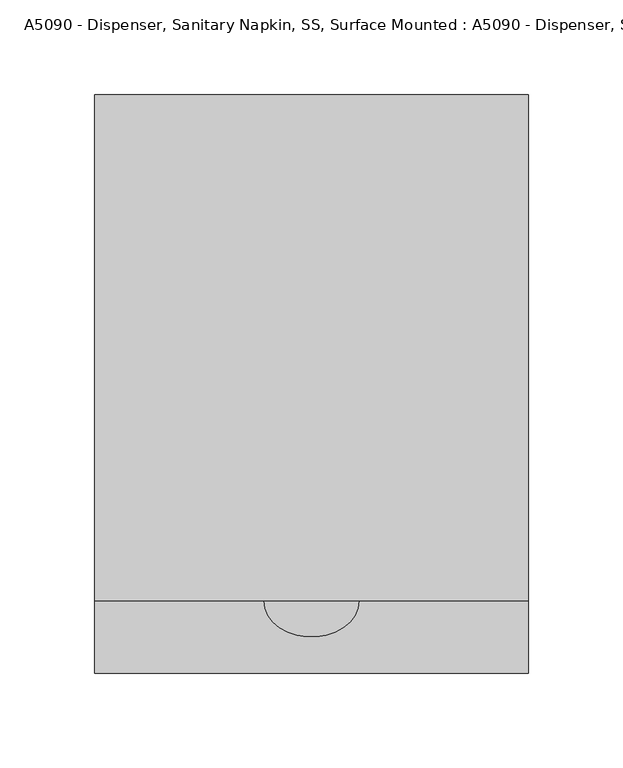
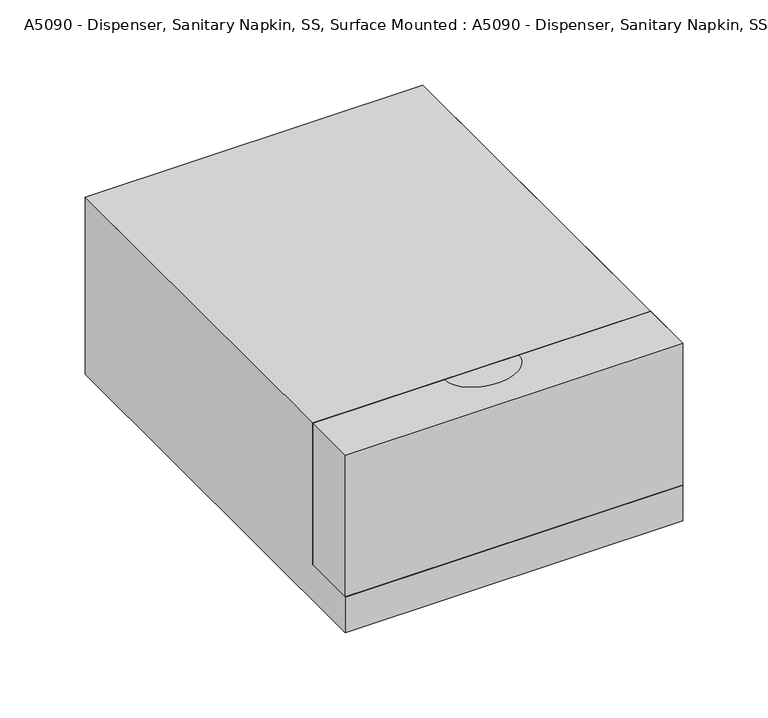
"""IFC4 building model written with IfcOpenShell, lengths in millimetres: proxy geometry, A5090 - Dispenser, Sanitary Napkin, SS, Surface Mounted : A5090 - Dispenser, Sanitary Napkin, SS, Surface Mounted."""

from ifc_helpers import new_model, si_unit, point, frame, origin, origin_with_axes, place, context, project, spatial, polyline, ellipse_curve, trimmed, outline, extrude, source, transform, mapped, element, save
from ifc_brep_helpers import plane_surface, extruded_surface, advanced_brep


def a5090_dispenser_sanitary_napkin_ss_surface_mounted_a5090_b2da7b39(model_context):
    return source(origin(), model_context, "Body", "SolidModel", [
        extrude(outline(polyline([(0.0, 127.0), (0.0, 0.0), (-304.8, 0.0), (-304.8, 25.4), (-266.7, 25.4), (-266.7, 127.0), (0.0, 127.0)])), frame((-114.3, 0.0, 0.0), z_axis=(1.0, 0.0, 0.0), x_axis=(0.0, 1.0, 0.0)), (0.0, 0.0, 1.0), 228.6),
        advanced_brep(
        [(114.3, -304.8, 127.0), (114.3, -266.7, 127.0), (25.4, -266.7, 127.0), (-25.4, -266.7, 127.0), (-114.3, -266.7, 127.0), (-114.3, -304.8, 127.0), (114.3, -304.8, 25.4), (-114.3, -304.8, 25.4), (-114.3, -266.7, 25.4), (-25.4, -266.7, 25.4), (25.4, -266.7, 25.4), (114.3, -266.7, 25.4)],
        [
            (0, 1),
            (1, 2),
            (2, 3, ellipse_curve(frame((0.0, -266.7, 127.0), z_axis=(0.0, 0.0, -1.0), x_axis=(1.0, 0.0, 0.0)), 25.4, 19.05)),
            (3, 4),
            (4, 5),
            (5, 0),
            (6, 7),
            (7, 8),
            (8, 9),
            (9, 10, ellipse_curve(frame((0.0, -266.7, 25.4), z_axis=(0.0, 0.0, 1.0), x_axis=(1.0, 0.0, 0.0)), 25.4, 19.05)),
            (10, 11),
            (11, 6),
            (5, 7),
            (6, 0),
            (4, 8),
            (3, 9),
            (2, 10),
            (1, 11),
        ],
        [
            plane_surface(frame((-114.3, -304.8, 127.0), z_axis=(0.0, 0.0, 1.0), x_axis=(-1.0, 0.0, 0.0))),
            plane_surface(frame((-114.3, -304.8, 25.4), z_axis=(0.0, 0.0, -1.0), x_axis=(1.0, 0.0, 0.0))),
            plane_surface(frame((114.3, -304.8, 127.0), z_axis=(0.0, -1.0, 0.0), x_axis=(0.0, 0.0, -1.0))),
            plane_surface(frame((-114.3, -304.8, 127.0), z_axis=(-1.0, 0.0, 0.0), x_axis=(0.0, 0.0, -1.0))),
            plane_surface(frame((-114.3, -266.7, 127.0), z_axis=(0.0, 1.0, 0.0), x_axis=(0.0, 0.0, -1.0))),
            extruded_surface(trimmed(ellipse_curve(frame((0.0, -266.7, 25.4), z_axis=(0.0, 0.0, 1.0), x_axis=(1.0, 0.0, 0.0)), 25.4, 19.05), [point((-25.4, -266.7, 25.4))], [point((25.4, -266.7, 25.4))], True, "CARTESIAN"), (0.0, 0.0, -101.6), 101.6),
            plane_surface(frame((25.4, -266.7, 127.0), z_axis=(0.0, 1.0, 0.0), x_axis=(0.0, 0.0, -1.0))),
            plane_surface(frame((114.3, -266.7, 127.0), z_axis=(1.0, 0.0, 0.0), x_axis=(0.0, 0.0, -1.0))),
        ],
        [
            (0, [[1, 2, 3, 4, 5, 6]]),
            (1, [[7, 8, 9, 10, 11, 12]]),
            (2, [[13, -7, 14, -6]]),
            (3, [[15, -8, -13, -5]]),
            (4, [[16, -9, -15, -4]]),
            (5, [[17, -10, -16, -3]]),
            (6, [[18, -11, -17, -2]]),
            (7, [[-14, -12, -18, -1]]),
        ],
    ),
        extrude(outline(polyline([(114.3, -304.8), (-114.3, -304.8), (-114.3, 0.0), (114.3, 0.0), (114.3, -304.8)])), origin_with_axes(), (0.0, 0.0, 1.0), 127.0),
    ])


if __name__ == "__main__":
    model = new_model("IFC4")
    model_context = context("Model", 3, world=origin())
    ifc_project = project(units=[si_unit("LENGTHUNIT", "METRE", prefix="MILLI")], contexts=[model_context])
    site = spatial("IfcSite", under=ifc_project)
    building = spatial("IfcBuilding", under=site)
    placement = place(None, origin())
    a5090_dispenser_sanitary_napkin_ss_surface_mounted_a5090_shape = a5090_dispenser_sanitary_napkin_ss_surface_mounted_a5090_b2da7b39(model_context)
    element("IfcBuildingElementProxy", 1, Name="A5090 - Dispenser, Sanitary Napkin, SS, Surface Mounted : A5090 - Dispenser, Sanitary Napkin, SS, Surface Mounted", ObjectType="A5090 - Dispenser, Sanitary Napkin, SS, Surface Mounted : A5090 - Dispenser, Sanitary Napkin, SS, Surface Mounted", at=placement, inside=building, context=model_context, shape_type="MappedRepresentation", body=[
        mapped(a5090_dispenser_sanitary_napkin_ss_surface_mounted_a5090_shape, transform((0.0, 0.0, 0.0), x_axis=(1.0, 0.0, 0.0), y_axis=(0.0, 1.0, 0.0), z_axis=(0.0, 0.0, 1.0))),
    ])
    save(model, "model.ifc")

# Revit data of these elements
# Type "A5090 - Dispenser, Sanitary Napkin, SS, Surface Mounted : A5090 - Dispenser, Sanitary Napkin, SS, Surface Mounted"
#   Watts2 = "0"
#   Watts1 = "0"
#   Unit_Issue = "EA"
#   UTIL_6_Misc = "-"
#   UTIL_5_NonMedGas = "-"
#   UTIL_4_MiscGas = "-"
#   UTIL_3_MedGas = "-"
#   UTIL_2_Elec = "-"
#   UTIL_1_WaterDrain = "-"
#   Nomenclature = "Disposal, Sanitary Napkin, SS, Surface Mounted"
#   NSN = "7240"
#   Location [instance default] = ""
#   JSN = "A5090"
#   Fund_Source_VA = "-"
#   Fund_Source_Navy = "-"
#   Fund_Source_Army = "-"
#   Fund_Source_AF = "-"
#   ELEC_Volts2 = "0"
#   ELEC_Volts1 = "0"
#   ELEC_Phase2 = "0"
#   ELEC_Phase1 = "0"
#   ELEC_HertzSwitch = "0"
#   ELEC_HertzDependent = "0"
#   ELEC_Hertz = "0"
#   ELEC_Amps2 = "0"
#   ELEC_Amps1 = "0"
#   DetailDescription = "A surface mounted, satin finish stainless steel, sanitary napkin disposal. Disposal features a flip-up cover, secured to the container by a heavy duty stainless steel piano-hinge. Disposal may be secured to wall or toilet partition. For general purpose use in female toilet stalls or rooms and uni-sex toilet rooms."
#   CAT_VA = "A"
#   CAT_Navy = "A"
#   CAT_IHS = "-"
#   CAT_Army = "A"
#   CAT_AF = "A"
#   BTUperhour = "0"
#   Weight_IP = 4
#   Default Elevation = 1' - 0"
#   DIM_Width_IP = 0' - 9"
#   DIM_Height_IP = 1' - 0"
#   DIM_Depth_IP = 0' - 5"
#   Assembly Code = ""
# Element 1 (IfcBuildingElementProxy, "A5090 - Dispenser, Sanitary Napkin, SS, Surface Mounted : A5090 - Dispenser, Sanitary Napkin, SS, Surface Mounted")
#   Location = "TLTS2"
#   Materials on its faces: "EquipSpace"
# Materials
#   "EquipSpace": class "Unassigned", colour RGB 221 217 195, transparency 0.5
